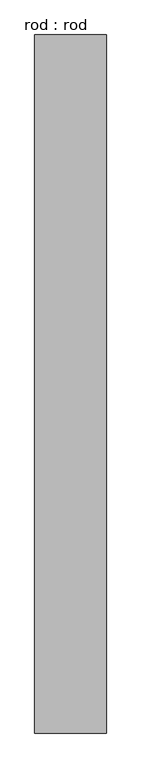
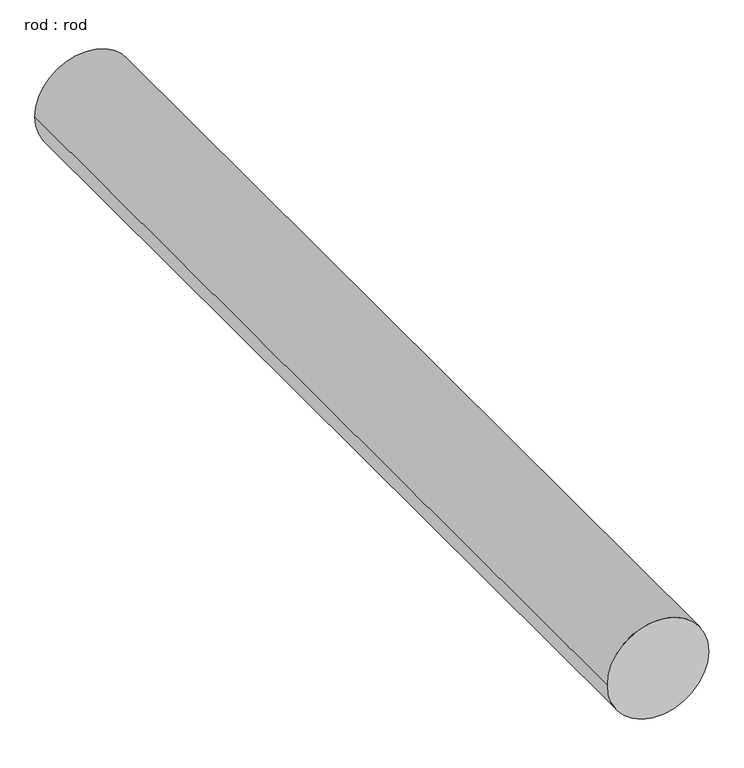
"""IFC4 building model written with IfcOpenShell, lengths in millimetres: proxy geometry, rod : rod."""

from ifc_helpers import new_model, si_unit, point, frame, frame_2d, origin, place, context, project, spatial, circle_curve, trimmed, segment, composite_curve, outline, extrude, source, transform, mapped, element, save


def rod_rod_82f8b94b(model_context):
    return source(origin(), model_context, "Body", "SweptSolid", [
        extrude(outline(composite_curve([segment(trimmed(circle_curve(frame_2d((0.0108462, 0.0)), 200.0), [point((0.0108462, 200.0))], [point((0.0108462, -200.0))], False, "CARTESIAN"), True, "CONTINUOUS"), segment(trimmed(circle_curve(frame_2d((0.0108462, 0.0)), 200.0), [point((0.0108462, -200.0))], [point((0.0108462, 200.0))], False, "CARTESIAN"), True, "CONTINUOUS")], self_intersect=False)), frame((0.0, 2143.175782, 0.0), z_axis=(0.0, 1.0, 0.0), x_axis=(0.0, 0.0, 1.0)), (0.0, 0.0, 1.0), 3899.1056667),
    ])


if __name__ == "__main__":
    model = new_model("IFC4")
    model_context = context("Model", 3, world=origin())
    ifc_project = project(units=[si_unit("LENGTHUNIT", "METRE", prefix="MILLI")], contexts=[model_context])
    site = spatial("IfcSite", under=ifc_project)
    building = spatial("IfcBuilding", under=site)
    placement = place(None, origin())
    rod_rod_shape = rod_rod_82f8b94b(model_context)
    element("IfcBuildingElementProxy", 1, Name="rod : rod", ObjectType="rod : rod", at=placement, inside=building, context=model_context, shape_type="MappedRepresentation", body=[
        mapped(rod_rod_shape, transform((0.0, 0.0, 0.0), x_axis=(1.0, 0.0, 0.0), y_axis=(0.0, 1.0, 0.0), z_axis=(0.0, 0.0, 1.0))),
    ])
    save(model, "model.ifc")

# Revit data of these elements
# Type "rod : rod"
#   Default Elevation = 0
